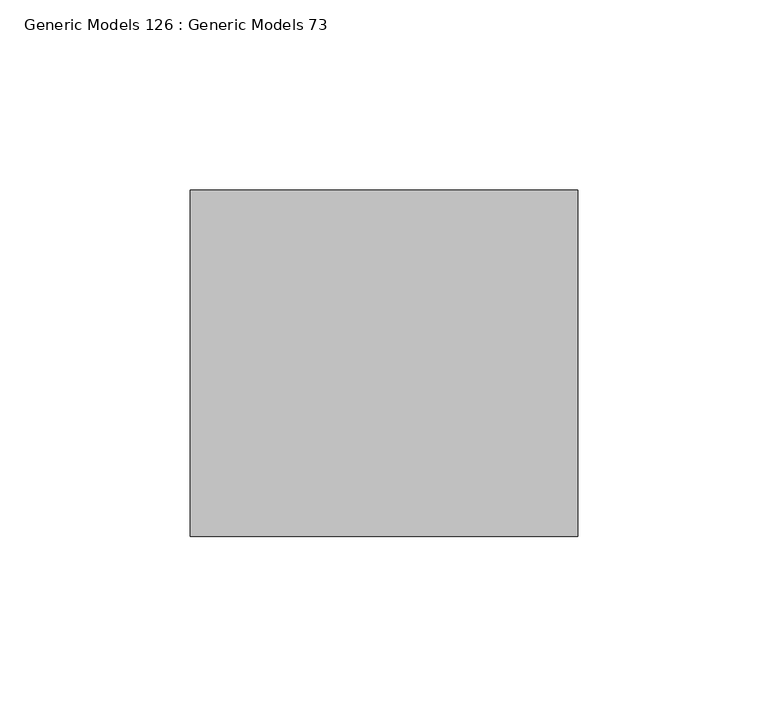
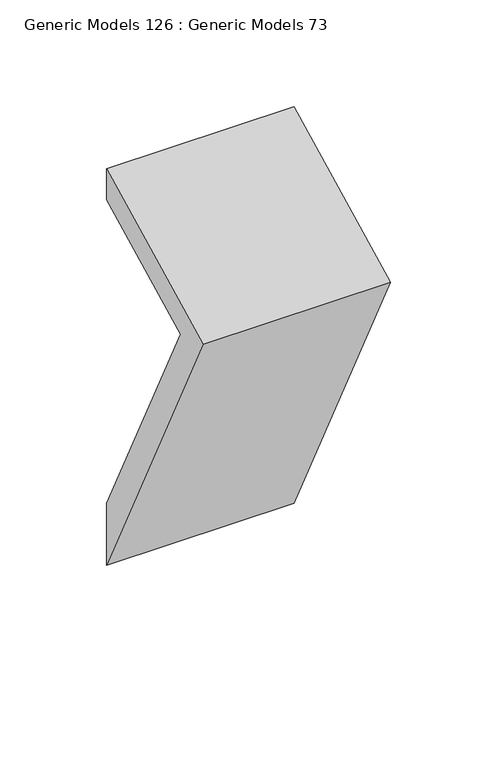
"""IFC4 building model written with IfcOpenShell, lengths in millimetres: proxy geometry, Generic Models 126 : Generic Models 73."""

from ifc_helpers import new_model, si_unit, frame, origin, place, context, project, spatial, polyline, outline, extrude, source, transform, mapped, element, save


def generic_models_126_generic_models_73_6a152cf2(model_context):
    return source(origin(), model_context, "Body", "SweptSolid", [
        extrude(outline(polyline([(35114.8094916, 268704.0255987), (35205.6832942, 268749.4625), (35205.6832942, 268731.7137104), (35136.1080391, 268696.9260829), (35205.6832942, 268557.7755726), (35205.6832942, 268522.2779935), (35114.8094916, 268704.0255987)])), frame((31924.6096032, 0.0, 0.0), z_axis=(1.0, 0.0, 0.0), x_axis=(0.0, 1.0, 0.0)), (0.0, 0.0, 1.0), 101.6),
    ])


if __name__ == "__main__":
    model = new_model("IFC4")
    model_context = context("Model", 3, world=origin())
    ifc_project = project(units=[si_unit("LENGTHUNIT", "METRE", prefix="MILLI")], contexts=[model_context])
    site = spatial("IfcSite", under=ifc_project)
    building = spatial("IfcBuilding", under=site)
    placement = place(None, origin())
    generic_models_126_generic_models_73_shape = generic_models_126_generic_models_73_6a152cf2(model_context)
    element("IfcBuildingElementProxy", 1, Name="Generic Models 126 : Generic Models 73", ObjectType="Generic Models 126 : Generic Models 73", at=placement, inside=building, context=model_context, shape_type="MappedRepresentation", body=[
        mapped(generic_models_126_generic_models_73_shape, transform((0.0, 0.0, 0.0), x_axis=(1.0, 0.0, 0.0), y_axis=(0.0, 1.0, 0.0), z_axis=(0.0, 0.0, 1.0))),
    ])
    save(model, "model.ifc")

# Revit data of these elements
# Element 1 (IfcBuildingElementProxy, "Generic Models 126 : Generic Models 73")
#   Materials on its faces: "L8 x 4 x 5/8 x 0'-4\" METAL ANGLE"
# Materials
#   "L8 x 4 x 5/8 x 0'-4\" METAL ANGLE": class "Metal", colour RGB 199 199 199, transparency 0, Description = "Carbon steel", Cost = 0
